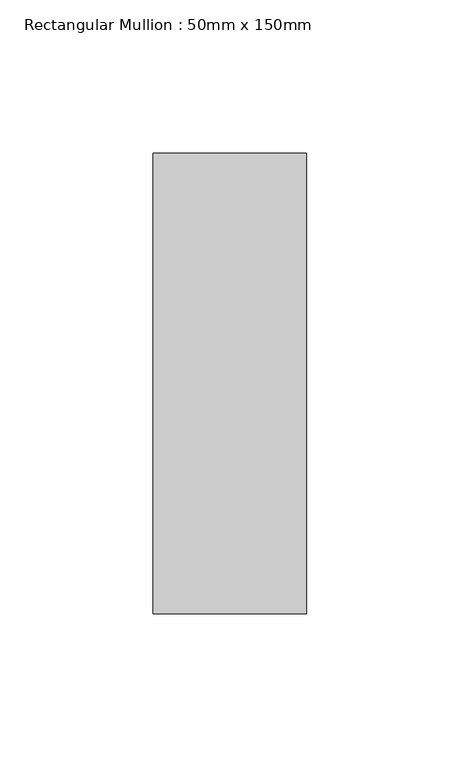
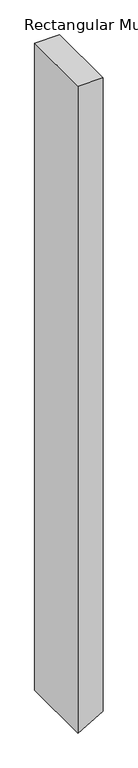
"""IFC4 building model written with IfcOpenShell, lengths in millimetres: member geometry, Rectangular Mullion : 50mm x 150mm."""

from ifc_helpers import new_model, si_unit, frame, origin, place, context, project, spatial, polyline, outline, extrude, source, transform, mapped, element, save


def rectangular_mullion_50mm_x_150mm_5374cabd(model_context):
    return source(origin(), model_context, "Body", "SweptSolid", [
        extrude(outline(polyline([(0.0, 25.0), (0.0, -25.0), (-1367.1254748, -25.0), (-1338.2579614, 25.0), (0.0, 25.0)])), frame((0.0, -75.0, 0.0), z_axis=(0.0, 1.0, 0.0), x_axis=(0.0, 0.0, 1.0)), (0.0, 0.0, 1.0), 150.0),
    ])


if __name__ == "__main__":
    model = new_model("IFC4")
    model_context = context("Model", 3, world=origin())
    ifc_project = project(units=[si_unit("LENGTHUNIT", "METRE", prefix="MILLI")], contexts=[model_context])
    site = spatial("IfcSite", under=ifc_project)
    building = spatial("IfcBuilding", under=site)
    placement = place(None, origin())
    rectangular_mullion_50mm_x_150mm_shape = rectangular_mullion_50mm_x_150mm_5374cabd(model_context)
    element("IfcMember", 1, ObjectType="Rectangular Mullion : 50mm x 150mm", at=placement, inside=building, context=model_context, shape_type="MappedRepresentation", body=[
        mapped(rectangular_mullion_50mm_x_150mm_shape, transform((0.0, 0.0, 0.0), x_axis=(1.0, 0.0, 0.0), y_axis=(0.0, 1.0, 0.0), z_axis=(0.0, 0.0, 1.0))),
    ])
    save(model, "model.ifc")

# Revit data of these elements
# Type "Rectangular Mullion : 50mm x 150mm"
#   built-in parameter 1007304 = 0.492126 (stored number, unit not read)
#   built-in parameter 1007301 = 0.082021 (stored number, unit not read)
#   built-in parameter 1007300 = 0.082021 (stored number, unit not read)
# Element 1 (IfcMember, "Rectangular Mullion : 50mm x 150mm")
#   Materials on its faces: "Aluminum"
# Materials
#   "Aluminum": class "Metal", colour RGB 247 247 247, transparency 0, Description = "Aluminum 6061", Cost = 0
